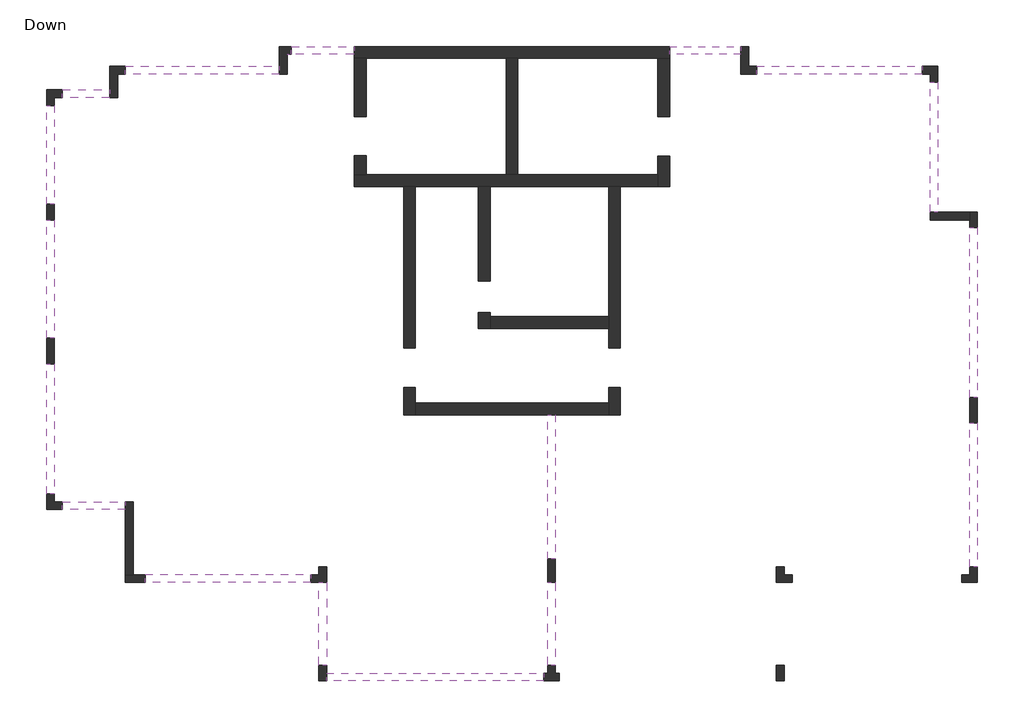
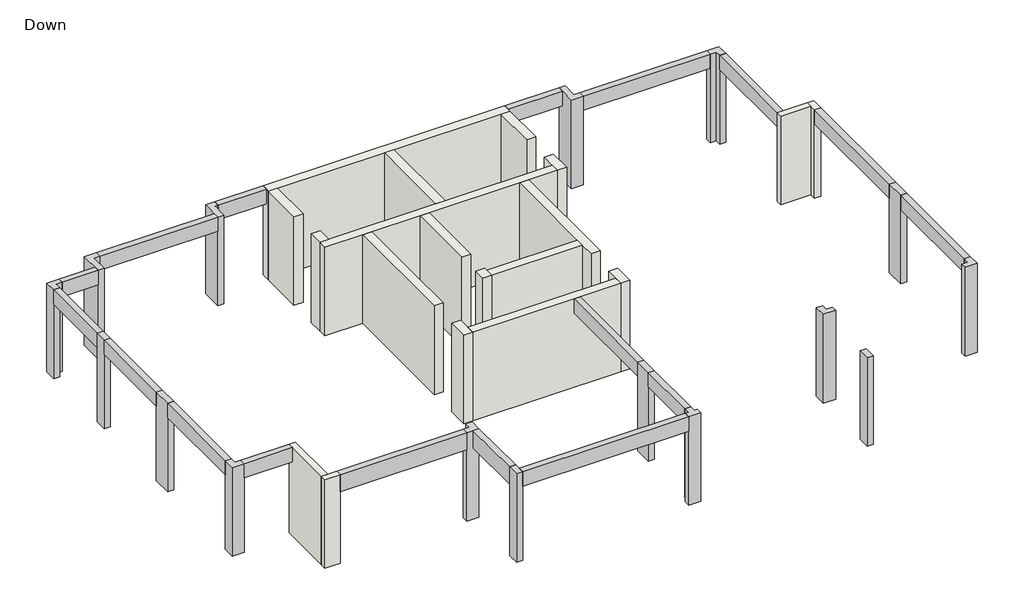
# One storey: 19 walls, 17 beams, 16 columns.
"""IFC4 building model written with IfcOpenShell, lengths in millimetres."""

from ifc_helpers import new_model, si_unit, frame, origin, origin_with_axes, place, context, project, spatial, polyline, outline, extrude, faceted_brep, element, save

model = new_model("IFC4")

# Units and contexts
model_context = context("Model", 3, world=origin())
ifc_project = project(units=[si_unit("LENGTHUNIT", "METRE", prefix="MILLI")], contexts=[model_context])

# Site, building, storey
site = spatial("IfcSite", under=ifc_project)
building = spatial("IfcBuilding", under=site)
storey = spatial("IfcBuildingStorey", under=building, Name="Down", Elevation=0.0)

# Beams
placement = place(None, origin())
element("IfcBeam", 1, ObjectType="Concrete Rectengular Beam : 20/50", at=placement, inside=storey, context=model_context, shape_type="Brep", body=[
    faceted_brep([(-10196.8748131, 3091.9867729, 3100.0), (-10196.8748131, 2891.9867729, 3100.0), (-6296.3457126, 2891.9867729, 3100.0), (-6296.3457126, 3091.9867729, 3100.0), (-10196.8748131, 3091.9867729, 2600.0), (-6296.3457126, 3091.9867729, 2600.0), (-10196.8748131, 2891.9867729, 2600.0), (-6296.3457126, 2891.9867729, 2600.0), (-10196.8748131, 2891.9867729, 2860.0)], [[[0, 1, 2, 3]], [[4, 0, 3, 5]], [[6, 4, 5, 7]], [[1, 8, 6, 7, 2]], [[1, 0, 4, 6, 8]], [[3, 2, 7, 5]]]),
])
element("IfcBeam", 2, ObjectType="Concrete Rectengular Beam : 20/50", at=placement, inside=storey, context=model_context, shape_type="Brep", body=[
    faceted_brep([(-11796.8748131, 2491.9867729, 3100.0), (-11796.8748131, 2291.9867729, 3100.0), (-10596.8748131, 2291.9867729, 3100.0), (-10596.8748131, 2491.9867729, 3100.0), (-11796.8748131, 2291.9867729, 2860.0), (-11796.8748131, 2291.9867729, 2600.0), (-10596.8748131, 2291.9867729, 2600.0), (-10596.8748131, 2291.9867729, 2860.0), (-11796.8748131, 2491.9867729, 2600.0), (-10596.8748131, 2491.9867729, 2600.0)], [[[0, 1, 2, 3]], [[2, 1, 4, 5, 6, 7]], [[5, 8, 9, 6]], [[8, 0, 3, 9]], [[1, 0, 8, 5, 4]], [[3, 2, 7, 6, 9]]]),
])
element("IfcBeam", 3, ObjectType="Concrete Rectengular Beam : 20/50", at=placement, inside=storey, context=model_context, shape_type="SweptSolid", body=[
    extrude(outline(polyline([(-11996.8748131, -407.4841265), (-12196.8748131, -407.4841265), (-12196.8748131, 2091.9867729), (-11996.8748131, 2091.9867729), (-11996.8748131, -407.4841265)])), frame((0.0, 0.0, 2600.0), z_axis=(0.0, 0.0, 1.0), x_axis=(1.0, 0.0, 0.0)), (0.0, 0.0, 1.0), 500.0),
])
element("IfcBeam", 4, ObjectType="Concrete Rectengular Beam : 20/50", at=placement, inside=storey, context=model_context, shape_type="SweptSolid", body=[
    extrude(outline(polyline([(-11996.8748131, -3806.4259255), (-12196.8748131, -3806.4259255), (-12196.8748131, -807.4841265), (-11996.8748131, -807.4841265), (-11996.8748131, -3806.4259255)])), frame((0.0, 0.0, 2600.0), z_axis=(0.0, 0.0, 1.0), x_axis=(1.0, 0.0, 0.0)), (0.0, 0.0, 1.0), 500.0),
])
element("IfcBeam", 5, ObjectType="Concrete Rectengular Beam : 20/50", at=placement, inside=storey, context=model_context, shape_type="SweptSolid", body=[
    extrude(outline(polyline([(-11996.8748131, -7755.6322747), (-12196.8748131, -7755.6322747), (-12196.8748131, -4456.4259255), (-11996.8748131, -4456.4259255), (-11996.8748131, -7755.6322747)])), frame((0.0, 0.0, 2600.0), z_axis=(0.0, 0.0, 1.0), x_axis=(1.0, 0.0, 0.0)), (0.0, 0.0, 1.0), 500.0),
])
element("IfcBeam", 6, ObjectType="Concrete Rectengular Beam : 20/50", at=placement, inside=storey, context=model_context, shape_type="Brep", body=[
    faceted_brep([(-11796.8748131, -7955.6322747, 3100.0), (-11796.8748131, -8155.6322747, 3100.0), (-10195.816612, -8155.6322747, 3100.0), (-10195.816612, -7955.6322747, 3100.0), (-10195.816612, -8155.6322747, 2600.0), (-11796.8748131, -8155.6322747, 2600.0), (-11796.8748131, -7955.6322747, 2600.0), (-10195.816612, -7955.6322747, 2600.0), (-10195.816612, -7955.6322747, 2860.0), (-11796.8748131, -7955.6322747, 2860.0)], [[[0, 1, 2, 3]], [[4, 2, 1, 5]], [[5, 6, 7, 4]], [[0, 3, 8, 7, 6, 9]], [[1, 0, 9, 6, 5]], [[3, 2, 4, 7, 8]]]),
])
element("IfcBeam", 7, ObjectType="Concrete Rectengular Beam : 20/50", at=placement, inside=storey, context=model_context, shape_type="Brep", body=[
    faceted_brep([(404.183388, -12504.8386239, 3100.0), (404.183388, -12304.8386239, 3100.0), (-5097.4039136, -12304.8386239, 3100.0), (-5097.4039136, -12504.8386239, 3100.0), (404.183388, -12304.8386239, 2600.0), (-5097.4039136, -12304.8386239, 2600.0), (-5097.4039136, -12304.8386239, 2860.0), (404.183388, -12504.8386239, 2600.0), (-5097.4039136, -12504.8386239, 2600.0)], [[[0, 1, 2, 3]], [[1, 4, 5, 6, 2]], [[4, 7, 8, 5]], [[7, 0, 3, 8]], [[1, 0, 7, 4]], [[2, 6, 5, 8, 3]]]),
])
element("IfcBeam", 8, ObjectType="Concrete Rectengular Beam : 20/50", at=placement, inside=storey, context=model_context, shape_type="SweptSolid", body=[
    extrude(outline(polyline([(11403.1251869, -9605.3677244), (11203.1251869, -9605.3677244), (11203.1251869, -5956.955026), (11403.1251869, -5956.955026), (11403.1251869, -9605.3677244)])), frame((0.0, 0.0, 2600.0), z_axis=(0.0, 0.0, 1.0), x_axis=(1.0, 0.0, 0.0)), (0.0, 0.0, 1.0), 500.0),
])
element("IfcBeam", 9, ObjectType="Concrete Rectengular Beam : 20/50", at=placement, inside=storey, context=model_context, shape_type="SweptSolid", body=[
    extrude(outline(polyline([(11403.1251869, -5306.955026), (11203.1251869, -5306.955026), (11203.1251869, -1006.4259255), (11403.1251869, -1006.4259255), (11403.1251869, -5306.955026)])), frame((0.0, 0.0, 2600.0), z_axis=(0.0, 0.0, 1.0), x_axis=(1.0, 0.0, 0.0)), (0.0, 0.0, 1.0), 500.0),
])
element("IfcBeam", 10, ObjectType="Concrete Rectengular Beam : 20/50", at=placement, inside=storey, context=model_context, shape_type="Brep", body=[
    faceted_brep([(10402.0669858, 2691.9867729, 3100.0), (10202.0669858, 2691.9867729, 3100.0), (10202.0669858, -606.4259255, 3100.0), (10402.0669858, -606.4259255, 3100.0), (10402.0669858, -606.4259255, 2600.0), (10402.0669858, 2691.9867729, 2600.0), (10202.0669858, 2691.9867729, 2600.0), (10202.0669858, -606.4259255, 2600.0), (10202.0669858, 2691.9867729, 2860.0), (10202.0669858, -606.4259255, 2860.0)], [[[0, 1, 2, 3]], [[3, 4, 5, 0]], [[6, 5, 4, 7]], [[2, 1, 8, 6, 7, 9]], [[1, 0, 5, 6, 8]], [[3, 2, 9, 7, 4]]]),
])
element("IfcBeam", 11, ObjectType="Concrete Rectengular Beam : 20/50", at=placement, inside=storey, context=model_context, shape_type="Brep", body=[
    faceted_brep([(10002.0669858, 2891.9867729, 3100.0), (10002.0669858, 3091.9867729, 3100.0), (5803.1251869, 3091.9867729, 3100.0), (5803.1251869, 2891.9867729, 3100.0), (10002.0669858, 3091.9867729, 2600.0), (5803.1251869, 3091.9867729, 2600.0), (10002.0669858, 2891.9867729, 2600.0), (5803.1251869, 2891.9867729, 2600.0), (5803.1251869, 2891.9867729, 2860.0), (10002.0669858, 2891.9867729, 2860.0)], [[[0, 1, 2, 3]], [[1, 4, 5, 2]], [[4, 6, 7, 5]], [[0, 3, 8, 7, 6, 9]], [[1, 0, 9, 6, 4]], [[3, 2, 5, 7, 8]]]),
])
element("IfcBeam", 12, ObjectType="Concrete Rectengular Beam : 20/50", at=placement, inside=storey, context=model_context, shape_type="SweptSolid", body=[
    extrude(outline(polyline([(704.183388, -12104.8386239), (504.183388, -12104.8386239), (504.183388, -10005.3677244), (704.183388, -10005.3677244), (704.183388, -12104.8386239)])), frame((0.0, 0.0, 2600.0), z_axis=(0.0, 0.0, 1.0), x_axis=(1.0, 0.0, 0.0)), (0.0, 0.0, 1.0), 500.0),
])
element("IfcBeam", 13, ObjectType="Concrete Rectengular Beam : 20/50", at=placement, inside=storey, context=model_context, shape_type="Brep", body=[
    faceted_brep([(-5996.3457126, 3591.4576724, 3100.0), (-5996.3457126, 3391.9867729, 3100.0), (-6096.3457126, 3391.9867729, 3100.0), (-6096.3457126, 3391.4576724, 3100.0), (-4395.816612, 3391.4576724, 3100.0), (-4395.816612, 3591.4576724, 3100.0), (-6096.3457126, 3391.4576724, 2860.0), (-6096.3457126, 3391.4576724, 2600.0), (-4395.816612, 3391.4576724, 2600.0), (-4395.816612, 3391.4576724, 2860.0), (-5996.3457126, 3391.9867729, 2600.0), (-5996.3457126, 3591.4576724, 2600.0), (-4395.816612, 3591.4576724, 2600.0), (-6096.3457126, 3391.9867729, 2600.0)], [[[0, 1, 2, 3, 4, 5]], [[3, 6, 7, 8, 9, 4]], [[10, 11, 12, 8, 7, 13]], [[11, 0, 5, 12]], [[10, 1, 0, 11]], [[1, 10, 13, 2]], [[2, 13, 7, 6, 3]], [[5, 4, 9, 8, 12]]]),
])
element("IfcBeam", 14, ObjectType="Concrete Rectengular Beam : 20/50", at=placement, inside=storey, context=model_context, shape_type="Brep", body=[
    faceted_brep([(3602.0669858, 3591.4576724, 3100.0), (3602.0669858, 3391.4576724, 3100.0), (5403.1251869, 3391.4576724, 3100.0), (5403.1251869, 3591.4576724, 3100.0), (3602.0669858, 3591.4576724, 2600.0), (5403.1251869, 3591.4576724, 2600.0), (3602.0669858, 3391.4576724, 2600.0), (5403.1251869, 3391.4576724, 2600.0), (3602.0669858, 3391.4576724, 2860.0), (5403.1251869, 3391.4576724, 2860.0)], [[[0, 1, 2, 3]], [[4, 0, 3, 5]], [[6, 4, 5, 7]], [[1, 8, 6, 7, 9, 2]], [[1, 0, 4, 6, 8]], [[3, 2, 9, 7, 5]]]),
])
element("IfcBeam", 15, ObjectType="Concrete Rectengular Beam : 20/50", at=placement, inside=storey, context=model_context, shape_type="Brep", body=[
    faceted_brep([(504.183388, -9405.3677244, 3100.0), (704.183388, -9405.3677244, 3100.0), (704.183388, -5755.6322747, 3100.0), (504.183388, -5755.6322747, 3100.0), (704.183388, -9405.3677244, 2600.0), (704.183388, -5755.6322747, 2600.0), (704.183388, -5755.6322747, 2860.0), (504.183388, -9405.3677244, 2600.0), (504.183388, -5755.6322747, 2600.0), (504.183388, -5755.6322747, 2860.0)], [[[0, 1, 2, 3]], [[1, 4, 5, 6, 2]], [[4, 7, 8, 5]], [[7, 0, 3, 9, 8]], [[1, 0, 7, 4]], [[3, 2, 6, 5, 8, 9]]]),
])
element("IfcBeam", 16, ObjectType="Concrete Rectengular Beam : 20/60", at=placement, inside=storey, context=model_context, shape_type="Brep", body=[
    faceted_brep([(-5497.4039136, -10005.3677244, 3100.0), (-5497.4039136, -9805.3677244, 3100.0), (-9695.2875115, -9805.3677244, 3100.0), (-9695.2875115, -10005.3677244, 3100.0), (-5497.4039136, -10005.3677244, 2500.0), (-9695.2875115, -10005.3677244, 2500.0), (-5497.4039136, -9805.3677244, 2500.0), (-9695.2875115, -9805.3677244, 2500.0), (-5497.4039136, -9805.3677244, 2860.0), (-9695.2875115, -9805.3677244, 2860.0)], [[[0, 1, 2, 3]], [[4, 0, 3, 5]], [[6, 4, 5, 7]], [[2, 1, 8, 6, 7, 9]], [[1, 0, 4, 6, 8]], [[3, 2, 9, 7, 5]]]),
])
element("IfcBeam", 17, ObjectType="Concrete Rectengular Beam : 20/60", at=placement, inside=storey, context=model_context, shape_type="Brep", body=[
    faceted_brep([(-5297.4039136, -12104.8386239, 3100.0), (-5097.4039136, -12104.8386239, 3100.0), (-5097.4039136, -10005.3677244, 3100.0), (-5297.4039136, -10005.3677244, 3100.0), (-5297.4039136, -12104.8386239, 2500.0), (-5297.4039136, -10005.3677244, 2860.0), (-5297.4039136, -10005.3677244, 2500.0), (-5097.4039136, -12104.8386239, 2500.0), (-5097.4039136, -10005.3677244, 2500.0), (-5097.4039136, -12104.8386239, 2860.0), (-5097.4039136, -10005.3677244, 2860.0)], [[[0, 1, 2, 3]], [[4, 0, 3, 5, 6]], [[7, 4, 6, 8]], [[2, 1, 9, 7, 8, 10]], [[1, 0, 4, 7, 9]], [[3, 2, 10, 8, 6, 5]]]),
])

# Columns
element("IfcColumn", 18, ObjectType="Concrete Rectengular Column : 20/40", at=placement, inside=storey, context=model_context, shape_type="Brep", body=[
    faceted_brep([(-5097.4039136, -12104.8386239, 0.0), (-5097.4039136, -12504.8386239, 0.0), (-5297.4039136, -12504.8386239, 0.0), (-5297.4039136, -12104.8386239, 0.0), (-5097.4039136, -12104.8386239, 3100.0), (-5097.4039136, -12304.8386239, 3100.0), (-5097.4039136, -12504.8386239, 3100.0), (-5297.4039136, -12504.8386239, 3100.0), (-5297.4039136, -12504.8386239, 2860.0), (-5297.4039136, -12104.8386239, 3100.0)], [[[0, 1, 2, 3]], [[4, 5, 6, 1, 0]], [[6, 7, 8, 2, 1]], [[7, 9, 3, 2, 8]], [[9, 4, 0, 3]], [[4, 9, 7, 6, 5]]]),
])
element("IfcColumn", 19, ObjectType="Concrete Rectengular Column : 20/40", at=placement, inside=storey, context=model_context, shape_type="SweptSolid", body=[
    extrude(outline(polyline([(-11996.8748131, -407.4841265), (-11996.8748131, -807.4841265), (-12196.8748131, -807.4841265), (-12196.8748131, -407.4841265), (-11996.8748131, -407.4841265)])), origin_with_axes(), (0.0, 0.0, 1.0), 3100.0),
])
element("IfcColumn", 20, ObjectType="Concrete Rectengular Column : 20/40", at=placement, inside=storey, context=model_context, shape_type="Brep", body=[
    faceted_brep([(6304.7124885, -12104.8386239, 0.0), (6504.7124885, -12104.8386239, 0.0), (6504.7124885, -12504.8386239, 0.0), (6304.7124885, -12504.8386239, 0.0), (6304.7124885, -12104.8386239, 3100.0), (6304.7124885, -12504.8386239, 3100.0), (6304.7124885, -12304.8386239, 3100.0), (6504.7124885, -12504.8386239, 3100.0), (6504.7124885, -12104.8386239, 3100.0)], [[[0, 1, 2, 3]], [[4, 0, 3, 5, 6]], [[5, 3, 2, 7]], [[7, 2, 1, 8]], [[8, 1, 0, 4]], [[4, 6, 5, 7, 8]]]),
])
element("IfcColumn", 21, ObjectType="Concrete Rectengular Column : 20/60", at=placement, inside=storey, context=model_context, shape_type="SweptSolid", body=[
    extrude(outline(polyline([(704.183388, -9405.3677244), (704.183388, -10005.3677244), (504.183388, -10005.3677244), (504.183388, -9405.3677244), (704.183388, -9405.3677244)])), origin_with_axes(), (0.0, 0.0, 1.0), 3100.0),
])
element("IfcColumn", 22, ObjectType="Concrete Rectengular Column : 20/65", at=placement, inside=storey, context=model_context, shape_type="SweptSolid", body=[
    extrude(outline(polyline([(-11996.8748131, -3806.4259255), (-11996.8748131, -4456.4259255), (-12196.8748131, -4456.4259255), (-12196.8748131, -3806.4259255), (-11996.8748131, -3806.4259255)])), origin_with_axes(), (0.0, 0.0, 1.0), 3100.0),
])
element("IfcColumn", 23, ObjectType="Concrete Rectengular Column : 20/65", at=placement, inside=storey, context=model_context, shape_type="SweptSolid", body=[
    extrude(outline(polyline([(11403.1251869, -5306.955026), (11403.1251869, -5956.955026), (11203.1251869, -5956.955026), (11203.1251869, -5306.955026), (11403.1251869, -5306.955026)])), origin_with_axes(), (0.0, 0.0, 1.0), 3100.0),
])
element("IfcColumn", 24, ObjectType="L Column : 40/40/20/20", at=placement, inside=storey, context=model_context, shape_type="Brep", body=[
    faceted_brep([(-5097.4039136, -10005.3677244, 0.0), (-5497.4039136, -10005.3677244, 0.0), (-5497.4039136, -9805.3677244, 0.0), (-5297.4039136, -9805.3677244, 0.0), (-5297.4039136, -9605.3677244, 0.0), (-5097.4039136, -9605.3677244, 0.0), (-5097.4039136, -10005.3677244, 3100.0), (-5297.4039136, -10005.3677244, 3100.0), (-5497.4039136, -10005.3677244, 3100.0), (-5497.4039136, -9805.3677244, 3100.0), (-5297.4039136, -9805.3677244, 3100.0), (-5297.4039136, -9805.3677244, 2860.0), (-5297.4039136, -9605.3677244, 3100.0), (-5297.4039136, -9605.3677244, 2860.0), (-5097.4039136, -9605.3677244, 3100.0), (-5097.4039136, -9605.3677244, 2860.0)], [[[0, 1, 2, 3, 4, 5]], [[6, 7, 8, 1, 0]], [[8, 9, 2, 1]], [[9, 10, 11, 3, 2]], [[10, 12, 13, 4, 3, 11]], [[12, 14, 15, 5, 4, 13]], [[14, 6, 0, 5, 15]], [[6, 14, 12, 10, 9, 8, 7]]]),
])
element("IfcColumn", 25, ObjectType="L Column : 40/40/20/20", at=placement, inside=storey, context=model_context, shape_type="Brep", body=[
    faceted_brep([(-12196.8748131, -8155.6322747, 0.0), (-12196.8748131, -7755.6322747, 0.0), (-11996.8748131, -7755.6322747, 0.0), (-11996.8748131, -7955.6322747, 0.0), (-11796.8748131, -7955.6322747, 0.0), (-11796.8748131, -8155.6322747, 0.0), (-12196.8748131, -8155.6322747, 3100.0), (-12196.8748131, -7755.6322747, 3100.0), (-11996.8748131, -7755.6322747, 3100.0), (-11996.8748131, -7955.6322747, 3100.0), (-11996.8748131, -7955.6322747, 2860.0), (-11796.8748131, -7955.6322747, 3100.0), (-11796.8748131, -8155.6322747, 3100.0)], [[[0, 1, 2, 3, 4, 5]], [[6, 7, 1, 0]], [[7, 8, 2, 1]], [[8, 9, 10, 3, 2]], [[9, 11, 4, 3, 10]], [[11, 12, 5, 4]], [[12, 6, 0, 5]], [[6, 12, 11, 9, 8, 7]]]),
])
element("IfcColumn", 26, ObjectType="L Column : 40/40/20/20", at=placement, inside=storey, context=model_context, shape_type="Brep", body=[
    faceted_brep([(-12196.8748131, 2491.9867729, 0.0), (-11796.8748131, 2491.9867729, 0.0), (-11796.8748131, 2291.9867729, 0.0), (-11996.8748131, 2291.9867729, 0.0), (-11996.8748131, 2091.9867729, 0.0), (-12196.8748131, 2091.9867729, 0.0), (-12196.8748131, 2491.9867729, 3100.0), (-11796.8748131, 2491.9867729, 3100.0), (-11796.8748131, 2291.9867729, 3100.0), (-11996.8748131, 2291.9867729, 3100.0), (-11996.8748131, 2291.9867729, 2860.0), (-11996.8748131, 2091.9867729, 3100.0), (-12196.8748131, 2091.9867729, 3100.0)], [[[0, 1, 2, 3, 4, 5]], [[6, 7, 1, 0]], [[7, 8, 2, 1]], [[8, 9, 10, 3, 2]], [[9, 11, 4, 3, 10]], [[11, 12, 5, 4]], [[12, 6, 0, 5]], [[6, 12, 11, 9, 8, 7]]]),
])
element("IfcColumn", 27, ObjectType="L Column : 40/40/20/20", at=placement, inside=storey, context=model_context, shape_type="Brep", body=[
    faceted_brep([(6304.7124885, -10005.3677244, 0.0), (6304.7124885, -9605.3677244, 0.0), (6504.7124885, -9605.3677244, 0.0), (6504.7124885, -9805.3677244, 0.0), (6704.7124885, -9805.3677244, 0.0), (6704.7124885, -10005.3677244, 0.0), (6304.7124885, -10005.3677244, 3100.0), (6704.7124885, -10005.3677244, 3100.0), (6704.7124885, -9805.3677244, 3100.0), (6504.7124885, -9805.3677244, 2860.0), (6504.7124885, -9805.3677244, 3100.0), (6504.7124885, -9605.3677244, 2860.0), (6504.7124885, -9605.3677244, 3100.0), (6304.7124885, -9605.3677244, 2860.0), (6304.7124885, -9605.3677244, 3100.0)], [[[0, 1, 2, 3, 4, 5]], [[6, 0, 5, 7]], [[7, 5, 4, 8]], [[8, 4, 3, 9, 10]], [[10, 9, 3, 2, 11, 12]], [[12, 11, 2, 1, 13, 14]], [[14, 13, 1, 0, 6]], [[6, 7, 8, 10, 12, 14]]]),
])
element("IfcColumn", 28, ObjectType="L Column : 40/40/20/20", at=placement, inside=storey, context=model_context, shape_type="Brep", body=[
    faceted_brep([(11403.1251869, -10005.3677244, 0.0), (11003.1251869, -10005.3677244, 0.0), (11003.1251869, -9805.3677244, 0.0), (11203.1251869, -9805.3677244, 0.0), (11203.1251869, -9605.3677244, 0.0), (11403.1251869, -9605.3677244, 0.0), (11403.1251869, -10005.3677244, 3100.0), (11003.1251869, -10005.3677244, 3100.0), (11003.1251869, -10005.3677244, 2500.0), (11003.1251869, -9805.3677244, 3100.0), (11003.1251869, -9805.3677244, 2500.0), (11203.1251869, -9805.3677244, 3100.0), (11203.1251869, -9805.3677244, 2860.0), (11203.1251869, -9605.3677244, 3100.0), (11403.1251869, -9605.3677244, 3100.0)], [[[0, 1, 2, 3, 4, 5]], [[6, 7, 8, 1, 0]], [[7, 9, 10, 2, 1, 8]], [[9, 11, 12, 3, 2, 10]], [[11, 13, 4, 3, 12]], [[13, 14, 5, 4]], [[14, 6, 0, 5]], [[6, 14, 13, 11, 9, 7]]]),
])
element("IfcColumn", 29, ObjectType="L Column : 40/40/20/20", at=placement, inside=storey, context=model_context, shape_type="Brep", body=[
    faceted_brep([(10402.0669858, 3091.9867729, 0.0), (10402.0669858, 2691.9867729, 0.0), (10202.0669858, 2691.9867729, 0.0), (10202.0669858, 2891.9867729, 0.0), (10002.0669858, 2891.9867729, 0.0), (10002.0669858, 3091.9867729, 0.0), (10402.0669858, 3091.9867729, 3100.0), (10402.0669858, 2691.9867729, 3100.0), (10202.0669858, 2691.9867729, 3100.0), (10202.0669858, 2891.9867729, 3100.0), (10202.0669858, 2891.9867729, 2860.0), (10002.0669858, 2891.9867729, 3100.0), (10002.0669858, 3091.9867729, 3100.0)], [[[0, 1, 2, 3, 4, 5]], [[6, 7, 1, 0]], [[7, 8, 2, 1]], [[8, 9, 10, 3, 2]], [[9, 11, 4, 3, 10]], [[11, 12, 5, 4]], [[12, 6, 0, 5]], [[6, 12, 11, 9, 8, 7]]]),
])
element("IfcColumn", 30, ObjectType="L Column : 70/40/20/20", at=placement, inside=storey, context=model_context, shape_type="Brep", body=[
    faceted_brep([(5403.1251869, 3591.9867729, 0.0), (5603.1251869, 3591.9867729, 0.0), (5603.1251869, 3091.9867729, 0.0), (5803.1251869, 3091.9867729, 0.0), (5803.1251869, 2891.9867729, 0.0), (5403.1251869, 2891.9867729, 0.0), (5403.1251869, 3591.9867729, 3100.0), (5603.1251869, 3591.9867729, 3100.0), (5603.1251869, 3091.9867729, 3100.0), (5803.1251869, 3091.9867729, 3100.0), (5803.1251869, 2891.9867729, 3100.0), (5403.1251869, 2891.9867729, 3100.0), (5403.1251869, 2891.9867729, 2860.0), (5403.1251869, 3391.4576724, 3100.0)], [[[0, 1, 2, 3, 4, 5]], [[6, 7, 1, 0]], [[7, 8, 2, 1]], [[8, 9, 3, 2]], [[9, 10, 4, 3]], [[10, 11, 12, 5, 4]], [[11, 13, 6, 0, 5, 12]], [[6, 13, 11, 10, 9, 8, 7]]]),
])
element("IfcColumn", 31, ObjectType="L Column : 70/40/30/20", at=placement, inside=storey, context=model_context, shape_type="Brep", body=[
    faceted_brep([(-6296.3457126, 3591.9867729, 0.0), (-5996.3457126, 3591.9867729, 0.0), (-5996.3457126, 3391.9867729, 0.0), (-6096.3457126, 3391.9867729, 0.0), (-6096.3457126, 2891.9867729, 0.0), (-6296.3457126, 2891.9867729, 0.0), (-6296.3457126, 3591.9867729, 3100.0), (-5996.3457126, 3591.9867729, 3100.0), (-5996.3457126, 3391.9867729, 3100.0), (-6096.3457126, 3391.9867729, 3100.0), (-6096.3457126, 3391.4576724, 3100.0), (-6096.3457126, 2891.9867729, 3100.0), (-6096.3457126, 2891.9867729, 2860.0), (-6296.3457126, 2891.9867729, 3100.0)], [[[0, 1, 2, 3, 4, 5]], [[6, 7, 1, 0]], [[7, 8, 2, 1]], [[8, 9, 3, 2]], [[9, 10, 11, 12, 4, 3]], [[11, 13, 5, 4, 12]], [[13, 6, 0, 5]], [[6, 13, 11, 10, 9, 8, 7]]]),
])
element("IfcColumn", 32, ObjectType="L Column : 80/40/20/20", at=placement, inside=storey, context=model_context, shape_type="Brep", body=[
    faceted_brep([(-10596.8748131, 3091.9867729, 0.0), (-10196.8748131, 3091.9867729, 0.0), (-10196.8748131, 2891.9867729, 0.0), (-10396.8748131, 2891.9867729, 0.0), (-10396.8748131, 2291.9867729, 0.0), (-10596.8748131, 2291.9867729, 0.0), (-10596.8748131, 3091.9867729, 3100.0), (-10196.8748131, 3091.9867729, 3100.0), (-10196.8748131, 2891.9867729, 3100.0), (-10396.8748131, 2891.9867729, 3100.0), (-10396.8748131, 2891.9867729, 2860.0), (-10396.8748131, 2291.9867729, 3100.0), (-10396.8748131, 2291.9867729, 2860.0), (-10596.8748131, 2291.9867729, 3100.0)], [[[0, 1, 2, 3, 4, 5]], [[6, 7, 1, 0]], [[7, 8, 2, 1]], [[8, 9, 10, 3, 2]], [[9, 11, 12, 4, 3, 10]], [[11, 13, 5, 4, 12]], [[13, 6, 0, 5]], [[6, 13, 11, 9, 8, 7]]]),
])
element("IfcColumn", 33, ObjectType="T Column : 40/40/20/20", at=placement, inside=storey, context=model_context, shape_type="Brep", body=[
    faceted_brep([(704.183388, -12104.8386239, 0.0), (704.183388, -12304.8386239, 0.0), (804.183388, -12304.8386239, 0.0), (804.183388, -12504.8386239, 0.0), (404.183388, -12504.8386239, 0.0), (404.183388, -12304.8386239, 0.0), (504.183388, -12304.8386239, 0.0), (504.183388, -12104.8386239, 0.0), (704.183388, -12104.8386239, 3100.0), (704.183388, -12304.8386239, 3100.0), (704.183388, -12304.8386239, 2860.0), (804.183388, -12304.8386239, 3100.0), (804.183388, -12504.8386239, 3100.0), (404.183388, -12504.8386239, 3100.0), (404.183388, -12304.8386239, 3100.0), (504.183388, -12304.8386239, 3100.0), (504.183388, -12304.8386239, 2860.0), (504.183388, -12104.8386239, 3100.0)], [[[0, 1, 2, 3, 4, 5, 6, 7]], [[8, 9, 10, 1, 0]], [[9, 11, 2, 1, 10]], [[11, 12, 3, 2]], [[12, 13, 4, 3]], [[13, 14, 5, 4]], [[14, 15, 16, 6, 5]], [[15, 17, 7, 6, 16]], [[17, 8, 0, 7]], [[8, 17, 15, 14, 13, 12, 11, 9]]]),
])

# Walls
element("IfcWall", 34, ObjectType="20", at=placement, inside=storey, context=model_context, shape_type="Brep", body=[
    faceted_brep([(-10195.816612, -7955.6322747, 0.0), (-10195.816612, -9805.3677244, 0.0), (-10195.816612, -9805.3677244, 3100.0), (-10195.816612, -7955.6322747, 3100.0), (-9995.816612, -7955.6322747, 0.0), (-9995.816612, -7955.6322747, 2860.0), (-9995.816612, -7955.6322747, 3100.0), (-9995.816612, -9805.3677244, 3100.0), (-9995.816612, -9805.3677244, 2860.0), (-9995.816612, -9805.3677244, 0.0)], [[[0, 1, 2, 3]], [[4, 5, 6, 7, 8, 9]], [[1, 0, 4, 9]], [[3, 2, 7, 6]], [[0, 3, 6, 5, 4]], [[2, 1, 9, 8, 7]]]),
])
element("IfcWall", 35, ObjectType="20", at=placement, inside=storey, context=model_context, shape_type="Brep", body=[
    faceted_brep([(-10195.816612, -10005.3677244, 0.0), (-9695.2875115, -10005.3677244, 0.0), (-9695.2875115, -10005.3677244, 2500.0), (-9695.2875115, -10005.3677244, 3100.0), (-10195.816612, -10005.3677244, 3100.0), (-10195.816612, -10005.3677244, 2860.0), (-10195.816612, -9805.3677244, 0.0), (-10195.816612, -9805.3677244, 3100.0), (-9995.816612, -9805.3677244, 3100.0), (-9695.2875115, -9805.3677244, 3100.0), (-9695.2875115, -9805.3677244, 2500.0), (-9695.2875115, -9805.3677244, 0.0), (-9995.816612, -9805.3677244, 0.0)], [[[0, 1, 2, 3, 4, 5]], [[6, 7, 8, 9, 10, 11, 12]], [[1, 0, 6, 12, 11]], [[3, 2, 1, 11, 10, 9]], [[4, 3, 9, 8, 7]], [[0, 5, 4, 7, 6]]]),
])
element("IfcWall", 36, ObjectType="20", at=placement, inside=storey, context=model_context, shape_type="Brep", body=[
    faceted_brep([(11403.1251869, -1006.4259255, 0.0), (11403.1251869, -606.4259255, 0.0), (11403.1251869, -606.4259255, 3100.0), (11403.1251869, -1006.4259255, 3100.0), (11403.1251869, -1006.4259255, 2600.0), (11203.1251869, -1006.4259255, 0.0), (11203.1251869, -1006.4259255, 2600.0), (11203.1251869, -1006.4259255, 3100.0), (11203.1251869, -806.4259255, 3100.0), (11203.1251869, -606.4259255, 3100.0), (11203.1251869, -606.4259255, 0.0), (11203.1251869, -806.4259255, 0.0)], [[[0, 1, 2, 3, 4]], [[5, 6, 7, 8, 9, 10, 11]], [[1, 0, 5, 11, 10]], [[3, 2, 9, 8, 7]], [[0, 4, 3, 7, 6, 5]], [[2, 1, 10, 9]]]),
])
element("IfcWall", 37, ObjectType="20", at=placement, inside=storey, context=model_context, shape_type="Brep", body=[
    faceted_brep([(11203.1251869, -606.4259255, 0.0), (10202.0669858, -606.4259255, 0.0), (10202.0669858, -606.4259255, 3100.0), (11203.1251869, -606.4259255, 3100.0), (11203.1251869, -806.4259255, 0.0), (11203.1251869, -806.4259255, 2860.0), (11203.1251869, -806.4259255, 3100.0), (10202.0669858, -806.4259255, 3100.0), (10202.0669858, -806.4259255, 2860.0), (10202.0669858, -806.4259255, 0.0)], [[[0, 1, 2, 3]], [[4, 5, 6, 7, 8, 9]], [[1, 0, 4, 9]], [[2, 1, 9, 8, 7]], [[3, 2, 7, 6]], [[0, 3, 6, 5, 4]]]),
])
element("IfcWall", 38, ObjectType="30", at=placement, inside=storey, context=model_context, shape_type="Brep", body=[
    faceted_brep([(-4395.816612, 3291.4576724, 0.0), (-4095.816612, 3291.4576724, 0.0), (-546.0811623, 3291.4576724, 0.0), (-246.0811623, 3291.4576724, 0.0), (3302.0669858, 3291.4576724, 0.0), (3602.0669858, 3291.4576724, 0.0), (3602.0669858, 3291.4576724, 3100.0), (3302.0669858, 3291.4576724, 3100.0), (-246.0811623, 3291.4576724, 3100.0), (-546.0811623, 3291.4576724, 3100.0), (-4095.816612, 3291.4576724, 3100.0), (-4395.816612, 3291.4576724, 3100.0), (-4395.816612, 3591.4576724, 0.0), (-4395.816612, 3591.4576724, 2600.0), (-4395.816612, 3591.4576724, 3100.0), (3602.0669858, 3591.4576724, 3100.0), (3602.0669858, 3591.4576724, 2600.0), (3602.0669858, 3591.4576724, 0.0), (3602.0669858, 3391.4576724, 3100.0), (-4395.816612, 3391.4576724, 3100.0)], [[[0, 1, 2, 3, 4, 5, 6, 7, 8, 9, 10, 11]], [[12, 13, 14, 15, 16, 17]], [[5, 4, 3, 2, 1, 0, 12, 17]], [[11, 10, 9, 8, 7, 6, 18, 15, 14, 19]], [[6, 5, 17, 16, 15, 18]], [[0, 11, 19, 14, 13, 12]]]),
])
element("IfcWall", 39, ObjectType="30", at=placement, inside=storey, context=model_context, shape_type="Brep", body=[
    faceted_brep([(3302.0669858, 3291.4576724, 0.0), (3302.0669858, 1816.8544978, 0.0), (3302.0669858, 1816.8544978, 2860.0), (3302.0669858, 1816.8544978, 3100.0), (3302.0669858, 3291.4576724, 3100.0), (3302.0669858, 3291.4576724, 2860.0), (3602.0669858, 3291.4576724, 0.0), (3602.0669858, 3291.4576724, 3100.0), (3602.0669858, 1816.8544978, 3100.0), (3602.0669858, 1816.8544978, 2860.0), (3602.0669858, 1816.8544978, 0.0), (3452.0669858, 1816.8544978, 3100.0)], [[[0, 1, 2, 3, 4, 5]], [[6, 7, 8, 9, 10]], [[1, 0, 6, 10]], [[3, 2, 1, 10, 9, 8, 11]], [[4, 3, 11, 8, 7]], [[0, 5, 4, 7, 6]]]),
])
element("IfcWall", 40, ObjectType="30", at=placement, inside=storey, context=model_context, shape_type="Brep", body=[
    faceted_brep([(3302.0669858, 811.5634925, 0.0), (3302.0669858, 343.3095243, 0.0), (3302.0669858, 43.3095243, 0.0), (3302.0669858, 43.3095243, 3100.0), (3302.0669858, 343.3095243, 3100.0), (3302.0669858, 811.5634925, 3100.0), (3302.0669858, 811.5634925, 2860.0), (3602.0669858, 811.5634925, 0.0), (3602.0669858, 811.5634925, 2860.0), (3602.0669858, 811.5634925, 3100.0), (3602.0669858, 43.3095243, 3100.0), (3602.0669858, 43.3095243, 2860.0), (3602.0669858, 43.3095243, 0.0), (3452.0669858, 811.5634925, 3100.0)], [[[0, 1, 2, 3, 4, 5, 6]], [[7, 8, 9, 10, 11, 12]], [[2, 1, 0, 7, 12]], [[5, 4, 3, 10, 9, 13]], [[0, 6, 5, 13, 9, 8, 7]], [[3, 2, 12, 11, 10]]]),
])
element("IfcWall", 41, ObjectType="30", at=placement, inside=storey, context=model_context, shape_type="Brep", body=[
    faceted_brep([(3302.0669858, 343.3095243, 0.0), (-246.0811623, 343.3095243, 0.0), (-546.0811623, 343.3095243, 0.0), (-4095.816612, 343.3095243, 0.0), (-4395.816612, 343.3095243, 0.0), (-4395.816612, 343.3095243, 3100.0), (-4095.816612, 343.3095243, 3100.0), (-546.0811623, 343.3095243, 3100.0), (-246.0811623, 343.3095243, 3100.0), (3302.0669858, 343.3095243, 3100.0), (3302.0669858, 343.3095243, 2860.0), (3302.0669858, 43.3095243, 0.0), (3302.0669858, 43.3095243, 3100.0), (2351.273335, 43.3095243, 3100.0), (2051.273335, 43.3095243, 3100.0), (-946.6102628, 43.3095243, 3100.0), (-1246.6102628, 43.3095243, 3100.0), (-2847.1393634, 43.3095243, 3100.0), (-3147.1393634, 43.3095243, 3100.0), (-4395.816612, 43.3095243, 3100.0), (-4395.816612, 43.3095243, 2860.0), (-4395.816612, 43.3095243, 0.0), (-3147.1393634, 43.3095243, 0.0), (-2847.1393634, 43.3095243, 0.0), (-1246.6102628, 43.3095243, 0.0), (-946.6102628, 43.3095243, 0.0), (2051.273335, 43.3095243, 0.0), (2351.273335, 43.3095243, 0.0)], [[[0, 1, 2, 3, 4, 5, 6, 7, 8, 9, 10]], [[11, 12, 13, 14, 15, 16, 17, 18, 19, 20, 21, 22, 23, 24, 25, 26, 27]], [[4, 3, 2, 1, 0, 11, 27, 26, 25, 24, 23, 22, 21]], [[9, 8, 7, 6, 5, 19, 18, 17, 16, 15, 14, 13, 12]], [[0, 10, 9, 12, 11]], [[5, 4, 21, 20, 19]]]),
])
element("IfcWall", 42, ObjectType="30", at=placement, inside=storey, context=model_context, shape_type="Brep", body=[
    faceted_brep([(-4095.816612, 343.3095243, 0.0), (-4095.816612, 817.9126989, 0.0), (-4095.816612, 817.9126989, 2860.0), (-4095.816612, 817.9126989, 3100.0), (-4095.816612, 343.3095243, 3100.0), (-4095.816612, 343.3095243, 2860.0), (-4395.816612, 343.3095243, 0.0), (-4395.816612, 343.3095243, 3100.0), (-4395.816612, 817.9126989, 3100.0), (-4395.816612, 817.9126989, 2860.0), (-4395.816612, 817.9126989, 0.0), (-4245.816612, 817.9126989, 3100.0)], [[[0, 1, 2, 3, 4, 5]], [[6, 7, 8, 9, 10]], [[1, 0, 6, 10]], [[3, 2, 1, 10, 9, 8, 11]], [[4, 3, 11, 8, 7]], [[0, 5, 4, 7, 6]]]),
])
element("IfcWall", 43, ObjectType="30", at=placement, inside=storey, context=model_context, shape_type="Brep", body=[
    faceted_brep([(-4095.816612, 1816.8544978, 0.0), (-4095.816612, 3291.4576724, 0.0), (-4095.816612, 3291.4576724, 2860.0), (-4095.816612, 3291.4576724, 3100.0), (-4095.816612, 1816.8544978, 3100.0), (-4095.816612, 1816.8544978, 2860.0), (-4395.816612, 1816.8544978, 0.0), (-4395.816612, 1816.8544978, 2860.0), (-4395.816612, 1816.8544978, 3100.0), (-4395.816612, 3291.4576724, 3100.0), (-4395.816612, 3291.4576724, 0.0), (-4245.816612, 1816.8544978, 3100.0)], [[[0, 1, 2, 3, 4, 5]], [[6, 7, 8, 9, 10]], [[1, 0, 6, 10]], [[4, 3, 9, 8, 11]], [[0, 5, 4, 11, 8, 7, 6]], [[3, 2, 1, 10, 9]]]),
])
element("IfcWall", 44, ObjectType="30", at=placement, inside=storey, context=model_context, shape_type="Brep", body=[
    faceted_brep([(-246.0811623, 343.3095243, 0.0), (-246.0811623, 3291.4576724, 0.0), (-246.0811623, 3291.4576724, 2860.0), (-246.0811623, 3291.4576724, 3100.0), (-246.0811623, 343.3095243, 3100.0), (-246.0811623, 343.3095243, 2860.0), (-546.0811623, 343.3095243, 0.0), (-546.0811623, 343.3095243, 2860.0), (-546.0811623, 343.3095243, 3100.0), (-546.0811623, 3291.4576724, 3100.0), (-546.0811623, 3291.4576724, 2860.0), (-546.0811623, 3291.4576724, 0.0)], [[[0, 1, 2, 3, 4, 5]], [[6, 7, 8, 9, 10, 11]], [[1, 0, 6, 11]], [[4, 3, 9, 8]], [[3, 2, 1, 11, 10, 9]], [[0, 5, 4, 8, 7, 6]]]),
])
element("IfcWall", 45, ObjectType="30", at=placement, inside=storey, context=model_context, shape_type="Brep", body=[
    faceted_brep([(-3147.1393634, 43.3095243, 0.0), (-3147.1393634, -4056.1613752, 0.0), (-3147.1393634, -4056.1613752, 2860.0), (-3147.1393634, -4056.1613752, 3100.0), (-3147.1393634, 43.3095243, 3100.0), (-3147.1393634, 43.3095243, 2860.0), (-2847.1393634, 43.3095243, 0.0), (-2847.1393634, 43.3095243, 3100.0), (-2847.1393634, -2356.6904757, 3100.0), (-2847.1393634, -4056.1613752, 3100.0), (-2847.1393634, -4056.1613752, 2860.0), (-2847.1393634, -4056.1613752, 0.0), (-2997.1393634, -4056.1613752, 3100.0)], [[[0, 1, 2, 3, 4, 5]], [[6, 7, 8, 9, 10, 11]], [[1, 0, 6, 11]], [[3, 2, 1, 11, 10, 9, 12]], [[4, 3, 12, 9, 8, 7]], [[0, 5, 4, 7, 6]]]),
])
element("IfcWall", 46, ObjectType="30", at=placement, inside=storey, context=model_context, shape_type="Brep", body=[
    faceted_brep([(-3147.1393634, -5057.2195763, 0.0), (-3147.1393634, -5755.6322747, 0.0), (-3147.1393634, -5755.6322747, 2860.0), (-3147.1393634, -5755.6322747, 3100.0), (-3147.1393634, -5057.2195763, 3100.0), (-3147.1393634, -5057.2195763, 2860.0), (-2847.1393634, -5057.2195763, 0.0), (-2847.1393634, -5057.2195763, 2860.0), (-2847.1393634, -5057.2195763, 3100.0), (-2847.1393634, -5455.6322747, 3100.0), (-2847.1393634, -5755.6322747, 3100.0), (-2847.1393634, -5755.6322747, 0.0), (-2847.1393634, -5455.6322747, 0.0), (-2997.1393634, -5057.2195763, 3100.0)], [[[0, 1, 2, 3, 4, 5]], [[6, 7, 8, 9, 10, 11, 12]], [[1, 0, 6, 12, 11]], [[4, 3, 10, 9, 8, 13]], [[0, 5, 4, 13, 8, 7, 6]], [[3, 2, 1, 11, 10]]]),
])
element("IfcWall", 47, ObjectType="30", at=placement, inside=storey, context=model_context, shape_type="Brep", body=[
    faceted_brep([(-2847.1393634, -5755.6322747, 0.0), (2053.3897372, -5755.6322747, 0.0), (2053.3897372, -5755.6322747, 3100.0), (704.183388, -5755.6322747, 3100.0), (504.183388, -5755.6322747, 3100.0), (-2847.1393634, -5755.6322747, 3100.0), (-2847.1393634, -5455.6322747, 0.0), (-2847.1393634, -5455.6322747, 2860.0), (-2847.1393634, -5455.6322747, 3100.0), (2053.3897372, -5455.6322747, 3100.0), (2053.3897372, -5455.6322747, 2860.0), (2053.3897372, -5455.6322747, 0.0)], [[[0, 1, 2, 3, 4, 5]], [[6, 7, 8, 9, 10, 11]], [[1, 0, 6, 11]], [[5, 4, 3, 2, 9, 8]], [[0, 5, 8, 7, 6]], [[2, 1, 11, 10, 9]]]),
])
element("IfcWall", 48, ObjectType="30", at=placement, inside=storey, context=model_context, shape_type="Brep", body=[
    faceted_brep([(2353.3897372, -5755.6322747, 0.0), (2353.3897372, -5055.6322747, 0.0), (2353.3897372, -5055.6322747, 2860.0), (2353.3897372, -5055.6322747, 3100.0), (2353.3897372, -5755.6322747, 3100.0), (2353.3897372, -5755.6322747, 2860.0), (2053.3897372, -5755.6322747, 0.0), (2053.3897372, -5755.6322747, 3100.0), (2053.3897372, -5455.6322747, 3100.0), (2053.3897372, -5055.6322747, 3100.0), (2053.3897372, -5055.6322747, 2860.0), (2053.3897372, -5055.6322747, 0.0), (2053.3897372, -5455.6322747, 0.0), (2201.273335, -5055.6322747, 3100.0)], [[[0, 1, 2, 3, 4, 5]], [[6, 7, 8, 9, 10, 11, 12]], [[1, 0, 6, 12, 11]], [[3, 2, 1, 11, 10, 9, 13]], [[4, 3, 13, 9, 8, 7]], [[0, 5, 4, 7, 6]]]),
])
element("IfcWall", 49, ObjectType="30", at=placement, inside=storey, context=model_context, shape_type="Brep", body=[
    faceted_brep([(2351.273335, -4056.1613752, 0.0), (2351.273335, 43.3095243, 0.0), (2351.273335, 43.3095243, 2860.0), (2351.273335, 43.3095243, 3100.0), (2351.273335, -4056.1613752, 3100.0), (2351.273335, -4056.1613752, 2860.0), (2051.273335, -4056.1613752, 0.0), (2051.273335, -4056.1613752, 2860.0), (2051.273335, -4056.1613752, 3100.0), (2051.273335, -3556.6904757, 3100.0), (2051.273335, -3256.6904757, 3100.0), (2051.273335, 43.3095243, 3100.0), (2051.273335, 43.3095243, 0.0), (2051.273335, -3256.6904757, 0.0), (2051.273335, -3556.6904757, 0.0), (2201.273335, -4056.1613752, 3100.0)], [[[0, 1, 2, 3, 4, 5]], [[6, 7, 8, 9, 10, 11, 12, 13, 14]], [[1, 0, 6, 14, 13, 12]], [[4, 3, 11, 10, 9, 8, 15]], [[0, 5, 4, 15, 8, 7, 6]], [[3, 2, 1, 12, 11]]]),
])
element("IfcWall", 50, ObjectType="30", at=placement, inside=storey, context=model_context, shape_type="Brep", body=[
    faceted_brep([(2051.273335, -3256.6904757, 0.0), (-946.6102628, -3256.6904757, 0.0), (-946.6102628, -3256.6904757, 3100.0), (2051.273335, -3256.6904757, 3100.0), (2051.273335, -3556.6904757, 0.0), (2051.273335, -3556.6904757, 2860.0), (2051.273335, -3556.6904757, 3100.0), (-946.6102628, -3556.6904757, 3100.0), (-946.6102628, -3556.6904757, 0.0)], [[[0, 1, 2, 3]], [[4, 5, 6, 7, 8]], [[1, 0, 4, 8]], [[3, 2, 7, 6]], [[0, 3, 6, 5, 4]], [[2, 1, 8, 7]]]),
])
element("IfcWall", 51, ObjectType="30", at=placement, inside=storey, context=model_context, shape_type="Brep", body=[
    faceted_brep([(-946.6102628, -3556.6904757, 0.0), (-946.6102628, -3256.6904757, 0.0), (-946.6102628, -3156.6904757, 0.0), (-946.6102628, -3156.6904757, 2860.0), (-946.6102628, -3156.6904757, 3100.0), (-946.6102628, -3256.6904757, 3100.0), (-946.6102628, -3556.6904757, 3100.0), (-1246.6102628, -3556.6904757, 0.0), (-1246.6102628, -3556.6904757, 2860.0), (-1246.6102628, -3556.6904757, 3100.0), (-1246.6102628, -3156.6904757, 3100.0), (-1246.6102628, -3156.6904757, 2860.0), (-1246.6102628, -3156.6904757, 0.0)], [[[0, 1, 2, 3, 4, 5, 6]], [[7, 8, 9, 10, 11, 12]], [[2, 1, 0, 7, 12]], [[4, 3, 2, 12, 11, 10]], [[6, 5, 4, 10, 9]], [[0, 6, 9, 8, 7]]]),
])
element("IfcWall", 52, ObjectType="30", at=placement, inside=storey, context=model_context, shape_type="Brep", body=[
    faceted_brep([(-946.6102628, -2356.6904757, 0.0), (-946.6102628, 43.3095243, 0.0), (-946.6102628, 43.3095243, 3100.0), (-946.6102628, -2356.6904757, 3100.0), (-946.6102628, -2356.6904757, 2860.0), (-1246.6102628, -2356.6904757, 0.0), (-1246.6102628, -2356.6904757, 3100.0), (-1246.6102628, 43.3095243, 3100.0), (-1246.6102628, 43.3095243, 0.0)], [[[0, 1, 2, 3, 4]], [[5, 6, 7, 8]], [[1, 0, 5, 8]], [[3, 2, 7, 6]], [[0, 4, 3, 6, 5]], [[2, 1, 8, 7]]]),
])

save(model, "model.ifc")

# Revit data of these elements
# Project information
#   Project Issue Date = "Issue Date"
#   Project Status = "Project Status"
#   Client Name = "לקוח"
#   Project Address = "Enter address here"
#   Project Name = "Project 006"
#   Project Number = "מספר פרויקט"
# Type "Concrete Rectengular Beam : 20/50"
#   Length [instance default] = 152.4 cm
#   b = 20 cm
#   h = 50 cm
#   Structural Material [instance default] = Concrete
#   Assembly Code = ""
# Type "Concrete Rectengular Beam : 20/60"
#   Length [instance default] = 152.4 cm
#   b = 20 cm
#   h = 60 cm
#   Structural Material [instance default] = Concrete
#   Assembly Code = ""
# Type "Concrete Rectengular Column : 20/40"
#   b = 20 cm
#   h = 40 cm
#   Structural Material [instance default] = Concrete
# Type "Concrete Rectengular Column : 20/60"
#   b = 20 cm
#   h = 60 cm
#   Structural Material [instance default] = Concrete
# Type "Concrete Rectengular Column : 20/65"
#   b = 20 cm
#   h = 65 cm
#   Structural Material [instance default] = Concrete
# Type "L Column : 40/40/20/20"
#   Small Length = 20 cm
#   Small Depth = 20 cm
#   Depth = 40 cm
#   Length = 40 cm
#   Centroid Y = 35 cm
#   Centroid X = 10 cm
#   Structural Material [instance default] = Concrete, Cast-in-Place gray
# Type "L Column : 70/40/20/20"
#   Small Length = 40 cm
#   Small Depth = 50 cm
#   Depth = 70 cm
#   Length = 20 cm
#   Centroid Y = 35 cm
#   Centroid X = 10 cm
#   Structural Material [instance default] = Concrete, Cast-in-Place gray
# Type "L Column : 70/40/30/20"
#   Small Length = 20 cm
#   Small Depth = 20 cm
#   Depth = 70 cm
#   Length = 30 cm
#   Centroid Y = 35 cm
#   Centroid X = 10 cm
#   Structural Material [instance default] = Concrete, Cast-in-Place gray
# Type "L Column : 80/40/20/20"
#   Small Length = 20 cm
#   Small Depth = 20 cm
#   Depth = 80 cm
#   Length = 40 cm
#   Centroid Y = 35 cm
#   Centroid X = 10 cm
#   Structural Material [instance default] = Concrete, Cast-in-Place gray
# Type "T Column : 40/40/20/20"
#   Small Length = 20 cm
#   Small Depth = 20 cm
#   Depth = 40 cm
#   Length = 40 cm
#   Centroid Y = 20 cm
#   Centroid X from Web = 10 cm
#   Centroid X from Flange = 20 cm
#   Structural Material [instance default] = Concrete, Cast-in-Place gray
# Type "20"
#   Layers, outside or top first: 20 cm "Concrete" (function 1)
# Type "30"
#   Layers, outside or top first: 30 cm "Concrete" (function 1)
# Element 1 (IfcBeam, "Concrete Rectengular Beam : 20/50")
#   Comments = ""
#   Mark = "B1"
#   SOFiSTiK_AMG_Comments = ""
#   SOFiSTiK_AMG_Scheduled = yes
#   SOFiSTiK_AMG_Adjusted = yes
#   Structural Material = Concrete
#   Phase Created = New Construction
#   Materials on its faces: "Concrete"
# Element 2 (IfcBeam, "Concrete Rectengular Beam : 20/50")
#   Comments = ""
#   Mark = "B2"
#   SOFiSTiK_AMG_Comments = ""
#   SOFiSTiK_AMG_Scheduled = yes
#   SOFiSTiK_AMG_Adjusted = yes
#   Structural Material = Concrete
#   Phase Created = New Construction
#   Materials on its faces: "Concrete"
# Element 3 (IfcBeam, "Concrete Rectengular Beam : 20/50")
#   Comments = ""
#   Mark = "B3"
#   SOFiSTiK_AMG_Comments = ""
#   SOFiSTiK_AMG_Scheduled = yes
#   SOFiSTiK_AMG_Adjusted = yes
#   Structural Material = Concrete
#   Phase Created = New Construction
#   Materials on its faces: "Concrete"
# Element 4 (IfcBeam, "Concrete Rectengular Beam : 20/50")
#   Comments = ""
#   Mark = "B4"
#   SOFiSTiK_AMG_Comments = ""
#   SOFiSTiK_AMG_Scheduled = yes
#   SOFiSTiK_AMG_Adjusted = yes
#   Structural Material = Concrete
#   Phase Created = New Construction
#   Materials on its faces: "Concrete"
# Element 5 (IfcBeam, "Concrete Rectengular Beam : 20/50")
#   Comments = ""
#   Mark = "B5"
#   SOFiSTiK_AMG_Comments = ""
#   SOFiSTiK_AMG_Scheduled = yes
#   SOFiSTiK_AMG_Adjusted = yes
#   Structural Material = Concrete
#   Phase Created = New Construction
#   Materials on its faces: "Concrete"
# Element 6 (IfcBeam, "Concrete Rectengular Beam : 20/50")
#   Comments = ""
#   Mark = "B6"
#   SOFiSTiK_AMG_Comments = ""
#   SOFiSTiK_AMG_Scheduled = yes
#   SOFiSTiK_AMG_Adjusted = yes
#   Structural Material = Concrete
#   Phase Created = New Construction
#   Materials on its faces: "Concrete"
# Element 7 (IfcBeam, "Concrete Rectengular Beam : 20/50")
#   Comments = ""
#   Mark = "B7"
#   SOFiSTiK_AMG_Comments = ""
#   SOFiSTiK_AMG_Scheduled = yes
#   SOFiSTiK_AMG_Adjusted = yes
#   Structural Material = Concrete
#   Phase Created = New Construction
#   Materials on its faces: "Concrete"
# Element 8 (IfcBeam, "Concrete Rectengular Beam : 20/50")
#   Comments = ""
#   Mark = "B9"
#   SOFiSTiK_AMG_Comments = ""
#   SOFiSTiK_AMG_Scheduled = yes
#   SOFiSTiK_AMG_Adjusted = yes
#   Structural Material = Concrete
#   Phase Created = New Construction
#   Materials on its faces: "Concrete"
# Element 9 (IfcBeam, "Concrete Rectengular Beam : 20/50")
#   Comments = ""
#   Mark = "B10"
#   SOFiSTiK_AMG_Comments = ""
#   SOFiSTiK_AMG_Scheduled = yes
#   SOFiSTiK_AMG_Adjusted = yes
#   Structural Material = Concrete
#   Phase Created = New Construction
#   Materials on its faces: "Concrete"
# Element 10 (IfcBeam, "Concrete Rectengular Beam : 20/50")
#   Comments = ""
#   Mark = "B11"
#   SOFiSTiK_AMG_Comments = ""
#   SOFiSTiK_AMG_Scheduled = yes
#   SOFiSTiK_AMG_Adjusted = yes
#   Structural Material = Concrete
#   Phase Created = New Construction
#   Materials on its faces: "Concrete"
# Element 11 (IfcBeam, "Concrete Rectengular Beam : 20/50")
#   Comments = ""
#   Mark = "B12"
#   SOFiSTiK_AMG_Comments = ""
#   SOFiSTiK_AMG_Scheduled = yes
#   SOFiSTiK_AMG_Adjusted = yes
#   Structural Material = Concrete
#   Phase Created = New Construction
#   Materials on its faces: "Concrete"
# Element 12 (IfcBeam, "Concrete Rectengular Beam : 20/50")
#   Comments = ""
#   Mark = "B13"
#   SOFiSTiK_AMG_Comments = ""
#   SOFiSTiK_AMG_Scheduled = yes
#   SOFiSTiK_AMG_Adjusted = yes
#   Structural Material = Concrete
#   Phase Created = New Construction
#   Materials on its faces: "Concrete"
# Element 13 (IfcBeam, "Concrete Rectengular Beam : 20/50")
#   Comments = ""
#   Mark = "B14"
#   SOFiSTiK_AMG_Comments = ""
#   SOFiSTiK_AMG_Scheduled = yes
#   SOFiSTiK_AMG_Adjusted = yes
#   Structural Material = Concrete
#   Phase Created = New Construction
#   Materials on its faces: "Concrete"
# Element 14 (IfcBeam, "Concrete Rectengular Beam : 20/50")
#   Comments = ""
#   Mark = "B15"
#   SOFiSTiK_AMG_Comments = ""
#   SOFiSTiK_AMG_Scheduled = yes
#   SOFiSTiK_AMG_Adjusted = yes
#   Structural Material = Concrete
#   Phase Created = New Construction
#   Materials on its faces: "Concrete"
# Element 15 (IfcBeam, "Concrete Rectengular Beam : 20/50")
#   Comments = ""
#   Mark = "B16"
#   SOFiSTiK_AMG_Comments = ""
#   SOFiSTiK_AMG_Scheduled = yes
#   SOFiSTiK_AMG_Adjusted = yes
#   Structural Material = Concrete
#   Phase Created = New Construction
#   Materials on its faces: "Concrete"
# Element 16 (IfcBeam, "Concrete Rectengular Beam : 20/60")
#   Comments = ""
#   Mark = "B17"
#   SOFiSTiK_AMG_Comments = ""
#   SOFiSTiK_AMG_Scheduled = yes
#   SOFiSTiK_AMG_Adjusted = yes
#   Structural Material = Concrete
#   Phase Created = New Construction
#   Materials on its faces: "Concrete"
# Element 17 (IfcBeam, "Concrete Rectengular Beam : 20/60")
#   Comments = ""
#   Mark = "B18"
#   SOFiSTiK_AMG_Comments = ""
#   SOFiSTiK_AMG_Scheduled = yes
#   SOFiSTiK_AMG_Adjusted = yes
#   Structural Material = Concrete
#   Phase Created = New Construction
#   Materials on its faces: "Concrete"
# Element 18 (IfcColumn, "Concrete Rectengular Column : 20/40")
#   Comments = ""
#   Mark = "C1"
#   SOFiSTiK_AMG_Comments = ""
#   SOFiSTiK_AMG_Scheduled = yes
#   SOFiSTiK_AMG_Adjusted = yes
#   Structural Material = Concrete
#   Phase Created = New Construction
#   Materials on its faces: "Concrete"
# Element 19 (IfcColumn, "Concrete Rectengular Column : 20/40")
#   Comments = ""
#   Mark = "C2"
#   SOFiSTiK_AMG_Comments = ""
#   SOFiSTiK_AMG_Scheduled = yes
#   SOFiSTiK_AMG_Adjusted = yes
#   Structural Material = Concrete
#   Phase Created = New Construction
#   Materials on its faces: "Concrete"
# Element 20 (IfcColumn, "Concrete Rectengular Column : 20/40")
#   Comments = ""
#   Mark = "C3"
#   SOFiSTiK_AMG_Comments = ""
#   SOFiSTiK_AMG_Scheduled = yes
#   SOFiSTiK_AMG_Adjusted = yes
#   Structural Material = Concrete
#   Phase Created = New Construction
#   Materials on its faces: "Concrete"
# Element 21 (IfcColumn, "Concrete Rectengular Column : 20/60")
#   Comments = ""
#   Mark = "C4"
#   SOFiSTiK_AMG_Comments = ""
#   SOFiSTiK_AMG_Scheduled = yes
#   SOFiSTiK_AMG_Adjusted = yes
#   Structural Material = Concrete
#   Phase Created = New Construction
#   Materials on its faces: "Concrete"
# Element 22 (IfcColumn, "Concrete Rectengular Column : 20/65")
#   Comments = ""
#   Mark = "C5"
#   SOFiSTiK_AMG_Comments = ""
#   SOFiSTiK_AMG_Scheduled = yes
#   SOFiSTiK_AMG_Adjusted = yes
#   Structural Material = Concrete
#   Phase Created = New Construction
#   Materials on its faces: "Concrete"
# Element 23 (IfcColumn, "Concrete Rectengular Column : 20/65")
#   Comments = ""
#   Mark = "C6"
#   SOFiSTiK_AMG_Comments = ""
#   SOFiSTiK_AMG_Scheduled = yes
#   SOFiSTiK_AMG_Adjusted = yes
#   Structural Material = Concrete
#   Phase Created = New Construction
#   Materials on its faces: "Concrete"
# Element 24 (IfcColumn, "L Column : 40/40/20/20")
#   Comments = ""
#   Mark = "C7"
#   SOFiSTiK_AMG_Comments = ""
#   SOFiSTiK_AMG_Scheduled = yes
#   SOFiSTiK_AMG_Adjusted = yes
#   Structural Material = Concrete
#   Phase Created = New Construction
# Element 25 (IfcColumn, "L Column : 40/40/20/20")
#   Comments = ""
#   Mark = "C8"
#   SOFiSTiK_AMG_Comments = ""
#   SOFiSTiK_AMG_Scheduled = yes
#   SOFiSTiK_AMG_Adjusted = yes
#   Structural Material = Concrete
#   Phase Created = New Construction
# Element 26 (IfcColumn, "L Column : 40/40/20/20")
#   Comments = ""
#   Mark = "C9"
#   SOFiSTiK_AMG_Comments = ""
#   SOFiSTiK_AMG_Scheduled = yes
#   SOFiSTiK_AMG_Adjusted = yes
#   Structural Material = Concrete
#   Phase Created = New Construction
# Element 27 (IfcColumn, "L Column : 40/40/20/20")
#   Comments = ""
#   Mark = "C10"
#   SOFiSTiK_AMG_Comments = ""
#   SOFiSTiK_AMG_Scheduled = yes
#   SOFiSTiK_AMG_Adjusted = yes
#   Structural Material = Concrete
#   Phase Created = New Construction
# Element 28 (IfcColumn, "L Column : 40/40/20/20")
#   Comments = ""
#   Mark = "C11"
#   SOFiSTiK_AMG_Comments = ""
#   SOFiSTiK_AMG_Scheduled = yes
#   SOFiSTiK_AMG_Adjusted = yes
#   Structural Material = Concrete
#   Phase Created = New Construction
# Element 29 (IfcColumn, "L Column : 40/40/20/20")
#   Comments = ""
#   Mark = "C12"
#   SOFiSTiK_AMG_Comments = ""
#   SOFiSTiK_AMG_Scheduled = yes
#   SOFiSTiK_AMG_Adjusted = yes
#   Structural Material = Concrete
#   Phase Created = New Construction
# Element 30 (IfcColumn, "L Column : 70/40/20/20")
#   Comments = ""
#   Mark = "C13"
#   SOFiSTiK_AMG_Comments = ""
#   SOFiSTiK_AMG_Scheduled = yes
#   SOFiSTiK_AMG_Adjusted = yes
#   Structural Material = Concrete
#   Phase Created = New Construction
# Element 31 (IfcColumn, "L Column : 70/40/30/20")
#   Comments = ""
#   Mark = "C14"
#   SOFiSTiK_AMG_Comments = ""
#   SOFiSTiK_AMG_Scheduled = yes
#   SOFiSTiK_AMG_Adjusted = yes
#   Structural Material = Concrete
#   Phase Created = New Construction
# Element 32 (IfcColumn, "L Column : 80/40/20/20")
#   Comments = ""
#   Mark = "C15"
#   SOFiSTiK_AMG_Comments = ""
#   SOFiSTiK_AMG_Scheduled = yes
#   SOFiSTiK_AMG_Adjusted = yes
#   Structural Material = Concrete
#   Phase Created = New Construction
# Element 33 (IfcColumn, "T Column : 40/40/20/20")
#   Comments = ""
#   Mark = "C16"
#   SOFiSTiK_AMG_Comments = ""
#   SOFiSTiK_AMG_Scheduled = yes
#   SOFiSTiK_AMG_Adjusted = yes
#   Structural Material = Concrete
#   Phase Created = New Construction
# Element 34 (IfcWall, "20")
#   Comments = ""
#   Mark = "W1"
#   SOFiSTiK_EdgeZones = "W1"
#   SOFiSTiK_AMG_Comments = ""
#   Top Offset = 0 cm
#   Base Offset = 0 cm
#   wall height = 310 cm
#   SOFiSTiK_AMG_Scheduled = yes
#   SOFiSTiK_AMG_Adjusted = yes
#   Phase Created = New Construction
#   Base Constraint = Down
#   Top Constraint = Typical Floor
#   Materials on its faces: "Concrete"
# Element 35 (IfcWall, "20")
#   Comments = ""
#   Mark = "W2"
#   SOFiSTiK_EdgeZones = "W2"
#   SOFiSTiK_AMG_Comments = ""
#   Top Offset = 0 cm
#   Base Offset = 0 cm
#   wall height = 310 cm
#   SOFiSTiK_AMG_Scheduled = yes
#   SOFiSTiK_AMG_Adjusted = yes
#   Phase Created = New Construction
#   Base Constraint = Down
#   Top Constraint = Typical Floor
#   Materials on its faces: "Concrete"
# Element 36 (IfcWall, "20")
#   Comments = ""
#   Mark = "W3"
#   SOFiSTiK_EdgeZones = "W3"
#   SOFiSTiK_AMG_Comments = ""
#   Top Offset = 0 cm
#   Base Offset = 0 cm
#   wall height = 310 cm
#   SOFiSTiK_AMG_Scheduled = yes
#   SOFiSTiK_AMG_Adjusted = yes
#   Phase Created = New Construction
#   Base Constraint = Down
#   Top Constraint = Typical Floor
#   Materials on its faces: "Concrete"
# Element 37 (IfcWall, "20")
#   Comments = ""
#   Mark = "W4"
#   SOFiSTiK_EdgeZones = "W4"
#   SOFiSTiK_AMG_Comments = ""
#   Top Offset = 0 cm
#   Base Offset = 0 cm
#   wall height = 310 cm
#   SOFiSTiK_AMG_Scheduled = yes
#   SOFiSTiK_AMG_Adjusted = yes
#   Phase Created = New Construction
#   Base Constraint = Down
#   Top Constraint = Typical Floor
#   Materials on its faces: "Concrete"
# Element 38 (IfcWall, "30")
#   Comments = ""
#   Mark = "W5"
#   SOFiSTiK_EdgeZones = "W5"
#   SOFiSTiK_AMG_Comments = ""
#   Top Offset = 0 cm
#   Base Offset = 0 cm
#   wall height = 310 cm
#   SOFiSTiK_AMG_Scheduled = yes
#   SOFiSTiK_AMG_Adjusted = yes
#   Phase Created = New Construction
#   Base Constraint = Down
#   Top Constraint = Typical Floor
#   Materials on its faces: "Concrete"
# Element 39 (IfcWall, "30")
#   Comments = ""
#   Mark = "W6"
#   SOFiSTiK_EdgeZones = "W6"
#   SOFiSTiK_AMG_Comments = ""
#   Top Offset = 0 cm
#   Base Offset = 0 cm
#   wall height = 310 cm
